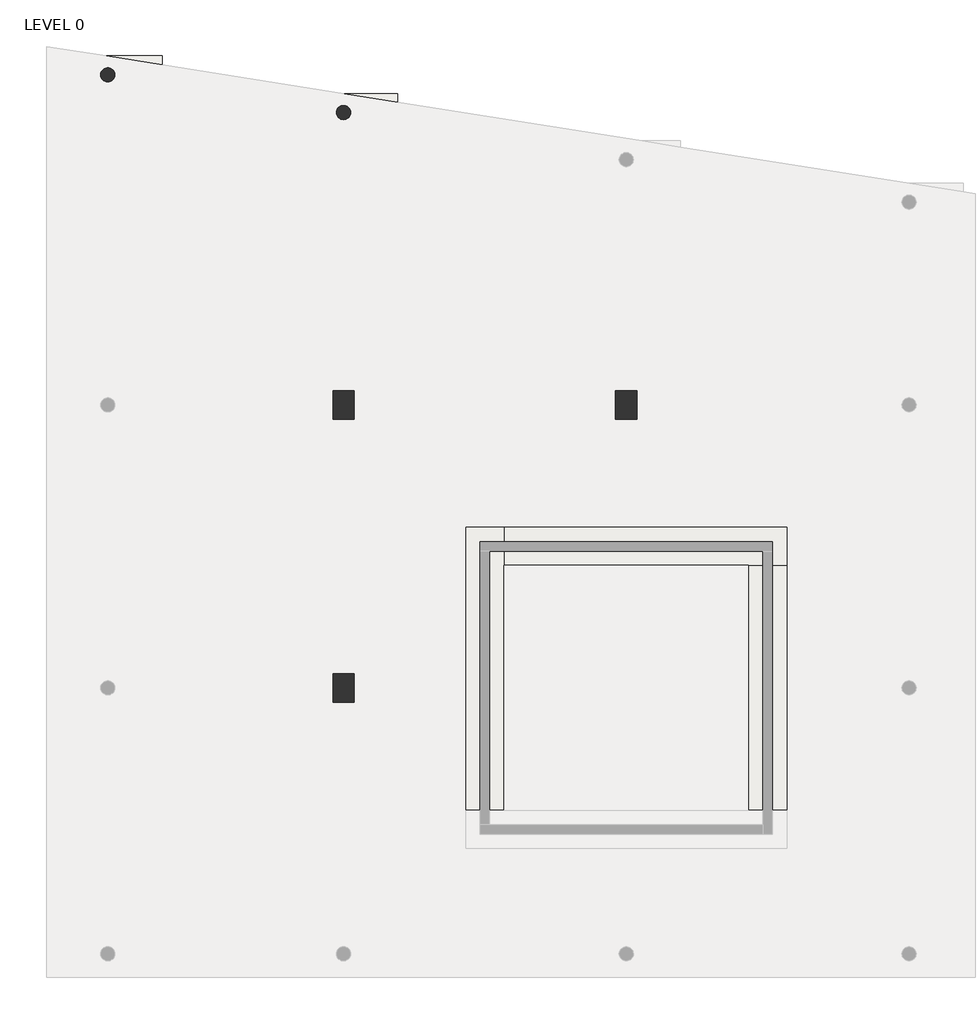
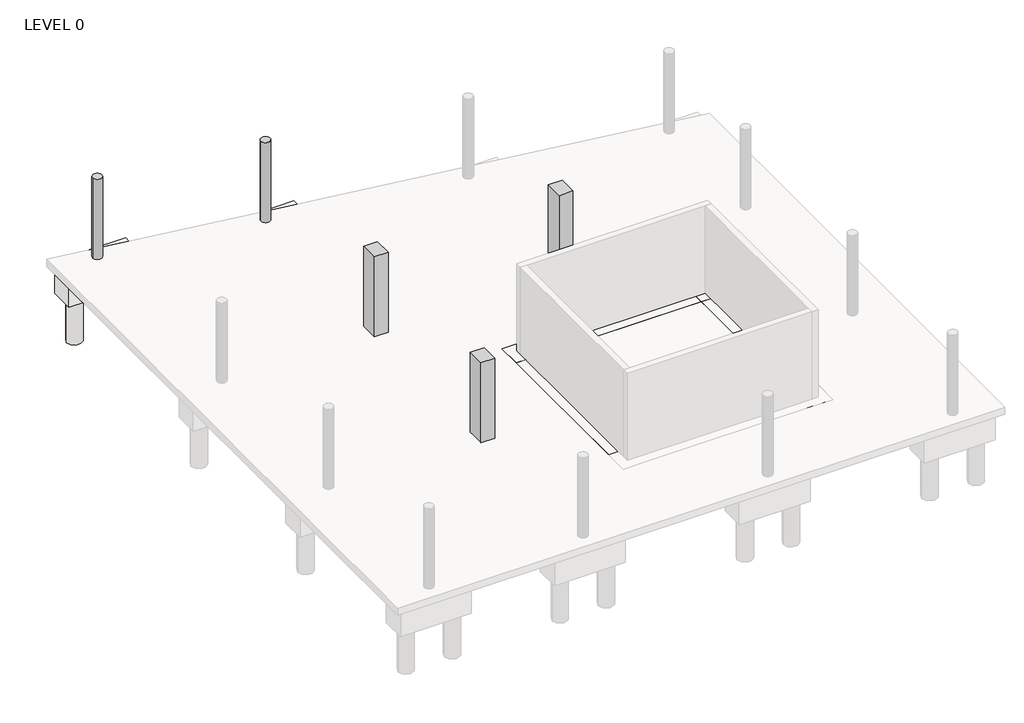
# One storey, part 2 of 3: 15 slabs, 5 columns, 3 footings.
"""IFC4 building model written with IfcOpenShell, lengths in millimetres."""

from ifc_helpers import new_model, si_unit, point, frame, frame_2d, origin, origin_with_axes, place, context, project, spatial, polyline, circle_curve, trimmed, segment, composite_curve, outline, extrude, faceted_brep, element, save
from ifc_brep_helpers import plane_surface, cylinder_surface, revolved_surface, advanced_brep

model = new_model("IFC4")

# Units and contexts
model_context = context("Model", 3, world=origin())
ifc_project = project(units=[si_unit("LENGTHUNIT", "METRE", prefix="MILLI")], contexts=[model_context])

# Site, building, storey
site = spatial("IfcSite", under=ifc_project)
building = spatial("IfcBuilding", under=site)
storey = spatial("IfcBuildingStorey", under=building, Name="LEVEL 0", Elevation=0.0)

# Columns
placement = place(None, origin())
element("IfcColumn", 1, ObjectType="BHm_StructuralColumns_ConcreteRound : 300 Ø RC COL", at=placement, inside=storey, context=model_context, shape_type="SweptSolid", body=[
    extrude(outline(composite_curve([segment(trimmed(circle_curve(frame_2d((-11075.1680269, 20840.7845261)), 150.0), [point((-11225.1680269, 20840.7845261))], [point((-10925.1680269, 20840.7845261))], False, "CARTESIAN"), True, "CONTINUOUS"), segment(trimmed(circle_curve(frame_2d((-11075.1680269, 20840.7845261)), 150.0), [point((-10925.1680269, 20840.7845261))], [point((-11225.1680269, 20840.7845261))], False, "CARTESIAN"), True, "CONTINUOUS")], self_intersect=False)), origin_with_axes(), (0.0, 0.0, 1.0), 2750.0),
])
element("IfcColumn", 2, ObjectType="BHm_StructuralColumns_ConcreteRound : 300 Ø RC COL", at=placement, inside=storey, context=model_context, shape_type="SweptSolid", body=[
    extrude(outline(composite_curve([segment(trimmed(circle_curve(frame_2d((-16075.1680269, 21640.7845261)), 150.0), [point((-16225.1680269, 21640.7845261))], [point((-15925.1680269, 21640.7845261))], False, "CARTESIAN"), True, "CONTINUOUS"), segment(trimmed(circle_curve(frame_2d((-16075.1680269, 21640.7845261)), 150.0), [point((-15925.1680269, 21640.7845261))], [point((-16225.1680269, 21640.7845261))], False, "CARTESIAN"), True, "CONTINUOUS")], self_intersect=False)), origin_with_axes(), (0.0, 0.0, 1.0), 2750.0),
])
element("IfcColumn", 3, ObjectType="BHm_StructuralColumns_ConcreteRectangular : 450x600 RC COL", at=placement, inside=storey, context=model_context, shape_type="SweptSolid", body=[
    extrude(outline(polyline([(-10850.1680269, 14940.7845261), (-10850.1680269, 14340.7845261), (-11300.1680269, 14340.7845261), (-11300.1680269, 14940.7845261), (-10850.1680269, 14940.7845261)])), origin_with_axes(), (0.0, 0.0, 1.0), 2750.0),
])
element("IfcColumn", 4, ObjectType="BHm_StructuralColumns_ConcreteRectangular : 450x600 RC COL", at=placement, inside=storey, context=model_context, shape_type="SweptSolid", body=[
    extrude(outline(polyline([(-10850.1680269, 8940.7845261), (-10850.1680269, 8340.7845261), (-11300.1680269, 8340.7845261), (-11300.1680269, 8940.7845261), (-10850.1680269, 8940.7845261)])), origin_with_axes(), (0.0, 0.0, 1.0), 2750.0),
])
element("IfcColumn", 5, ObjectType="BHm_StructuralColumns_ConcreteRectangular : 450x600 RC COL", at=placement, inside=storey, context=model_context, shape_type="SweptSolid", body=[
    extrude(outline(polyline([(-4850.1680269, 14940.7845261), (-4850.1680269, 14340.7845261), (-5300.1680269, 14340.7845261), (-5300.1680269, 14940.7845261), (-4850.1680269, 14940.7845261)])), origin_with_axes(), (0.0, 0.0, 1.0), 2750.0),
])

# Footings
element("IfcFooting", 6, ObjectType="Wall Foundation", at=placement, inside=storey, context=model_context, shape_type="Brep", body=[
    faceted_brep([(-7670.3680269, 5235.9845261, 0.0), (-7670.3680269, 6045.5845261, 0.0), (-7670.3680269, 11235.9845261, 0.0), (-7670.3680269, 12045.5845261, 0.0), (-8479.9680269, 12045.5845261, 0.0), (-8479.9680269, 5235.9845261, 0.0), (-8479.9680269, 5235.9845261, -500.0), (-8479.9680269, 5235.9845261, -250.0), (-8479.9680269, 12045.5845261, -250.0), (-8479.9680269, 12045.5845261, -500.0), (-7670.3680269, 5235.9845261, -500.0), (-7670.3680269, 12045.5845261, -500.0)], [[[0, 1, 2, 3, 4, 5]], [[6, 7, 5, 4, 8, 9]], [[10, 6, 9, 11]], [[0, 10, 11, 3, 2, 1]], [[4, 3, 11, 9, 8]], [[0, 5, 7, 6, 10]]]),
])
element("IfcFooting", 7, ObjectType="Wall Foundation", at=placement, inside=storey, context=model_context, shape_type="Brep", body=[
    faceted_brep([(-8479.9680269, 11235.9845261, 0.0), (-7670.3680269, 11235.9845261, 0.0), (-2479.9680269, 11235.9845261, 0.0), (-1670.3680269, 11235.9845261, 0.0), (-1670.3680269, 12045.5845261, 0.0), (-8479.9680269, 12045.5845261, 0.0), (-8479.9680269, 12045.5845261, -500.0), (-8479.9680269, 12045.5845261, -250.0), (-1670.3680269, 12045.5845261, -250.0), (-1670.3680269, 12045.5845261, -500.0), (-8479.9680269, 11235.9845261, -500.0), (-1670.3680269, 11235.9845261, -500.0)], [[[0, 1, 2, 3, 4, 5]], [[6, 7, 5, 4, 8, 9]], [[10, 6, 9, 11]], [[0, 10, 11, 3, 2, 1]], [[0, 5, 7, 6, 10]], [[4, 3, 11, 9, 8]]]),
])
element("IfcFooting", 8, ObjectType="Wall Foundation", at=placement, inside=storey, context=model_context, shape_type="Brep", body=[
    faceted_brep([(-2479.9680269, 12045.5845261, 0.0), (-2479.9680269, 11235.9845261, 0.0), (-2479.9680269, 6045.5845261, 0.0), (-2479.9680269, 5235.9845261, 0.0), (-1670.3680269, 5235.9845261, 0.0), (-1670.3680269, 12045.5845261, 0.0), (-1670.3680269, 12045.5845261, -500.0), (-1670.3680269, 12045.5845261, -250.0), (-1670.3680269, 5235.9845261, -250.0), (-1670.3680269, 5235.9845261, -500.0), (-2479.9680269, 12045.5845261, -500.0), (-2479.9680269, 5235.9845261, -500.0)], [[[0, 1, 2, 3, 4, 5]], [[6, 7, 5, 4, 8, 9]], [[10, 6, 9, 11]], [[0, 10, 11, 3, 2, 1]], [[0, 5, 7, 6, 10]], [[4, 3, 11, 9, 8]]]),
])

# Slabs
element("IfcSlab", 9, ObjectType="BHm_StructuralFoundations_RC-2PileCap : 500Ø R.C. 2-PILE CAP", at=placement, inside=storey, context=model_context, shape_type="AdvancedBrep", body=[
    advanced_brep(
    [(-9925.1680269, 15040.7845261, -1100.0), (-9925.1680269, 14240.7845261, -1100.0), (-12225.1680269, 14240.7845261, -1100.0), (-12225.1680269, 15040.7845261, -1100.0), (-12075.1680269, 14640.7845261, -1100.0), (-11575.1680269, 14640.7845261, -1100.0), (-10575.1680269, 14640.7845261, -1100.0), (-10075.1680269, 14640.7845261, -1100.0), (-12225.1680269, 15040.7845261, -250.0), (-9925.1680269, 15040.7845261, -250.0), (-12225.1680269, 14240.7845261, -250.0), (-9925.1680269, 14240.7845261, -250.0), (-10575.1680269, 14640.7845261, -1025.0), (-10075.1680269, 14640.7845261, -1025.0), (-12075.1680269, 14640.7845261, -1025.0), (-11575.1680269, 14640.7845261, -1025.0)],
    [
        (0, 1),
        (1, 2),
        (2, 3),
        (3, 0),
        (4, 5, circle_curve(frame((-11825.1680269, 14640.7845261, -1100.0), z_axis=(0.0, 0.0, 1.0), x_axis=(1.0, 0.0, 0.0)), 250.0)),
        (5, 4, circle_curve(frame((-11825.1680269, 14640.7845261, -1100.0), z_axis=(0.0, 0.0, 1.0), x_axis=(1.0, 0.0, 0.0)), 250.0)),
        (6, 7, circle_curve(frame((-10325.1680269, 14640.7845261, -1100.0), z_axis=(0.0, 0.0, 1.0), x_axis=(1.0, 0.0, 0.0)), 250.0)),
        (7, 6, circle_curve(frame((-10325.1680269, 14640.7845261, -1100.0), z_axis=(0.0, 0.0, 1.0), x_axis=(1.0, 0.0, 0.0)), 250.0)),
        (3, 8),
        (8, 9),
        (9, 0),
        (2, 10),
        (10, 8),
        (1, 11),
        (11, 10),
        (9, 11),
        (12, 13, circle_curve(frame((-10325.1680269, 14640.7845261, -1025.0), z_axis=(0.0, 0.0, -1.0), x_axis=(1.0, 0.0, 0.0)), 250.0)),
        (13, 12, circle_curve(frame((-10325.1680269, 14640.7845261, -1025.0), z_axis=(0.0, 0.0, -1.0), x_axis=(1.0, 0.0, 0.0)), 250.0)),
        (4, 14),
        (14, 15, circle_curve(frame((-11825.1680269, 14640.7845261, -1025.0), z_axis=(0.0, 0.0, 1.0), x_axis=(1.0, 0.0, 0.0)), 250.0)),
        (15, 5),
        (15, 14, circle_curve(frame((-11825.1680269, 14640.7845261, -1025.0), z_axis=(0.0, 0.0, 1.0), x_axis=(1.0, 0.0, 0.0)), 250.0)),
        (6, 12),
        (13, 7),
    ],
    [
        plane_surface(frame((-12225.1680269, 15040.7845261, -1100.0), z_axis=(0.0, 0.0, -1.0), x_axis=(1.0, 0.0, 0.0))),
        plane_surface(frame((-9925.1680269, 15040.7845261, 0.0), z_axis=(0.0, 1.0, 0.0), x_axis=(0.0, 0.0, -1.0))),
        plane_surface(frame((-12225.1680269, 15040.7845261, 0.0), z_axis=(-1.0, 0.0, 0.0), x_axis=(0.0, 0.0, -1.0))),
        plane_surface(frame((-12225.1680269, 14240.7845261, 0.0), z_axis=(0.0, -1.0, 0.0), x_axis=(0.0, 0.0, -1.0))),
        plane_surface(frame((-9925.1680269, 14240.7845261, 0.0), z_axis=(1.0, 0.0, 0.0), x_axis=(0.0, 0.0, -1.0))),
        plane_surface(frame((-11575.1680269, 14640.7845261, -1025.0), z_axis=(0.0, 0.0, -1.0), x_axis=(0.0, 1.0, 0.0))),
        revolved_surface(polyline([(-11575.1680269, 14640.7845261, -1025.0), (-11575.1680269, 14640.7845261, -1100.0)]), (-11825.1680269, 14640.7845261, -1100.0), (0.0, 0.0, 1.0)),
        revolved_surface(polyline([(-10075.1680269, 14640.7845261, -1025.0), (-10075.1680269, 14640.7845261, -1100.0)]), (-10325.1680269, 14640.7845261, 0.0), (0.0, 0.0, 1.0)),
        plane_surface(frame((2324.8319731, 15140.7845261, -250.0), z_axis=(0.0, 0.0, 1.0), x_axis=(0.0, -1.0, 0.0))),
    ],
    [
        (0, [[1, 2, 3, 4], [5, 6], [7, 8]]),
        (1, [[-4, 9, 10, 11]]),
        (2, [[-3, 12, 13, -9]]),
        (3, [[-2, 14, 15, -12]]),
        (4, [[-1, -11, 16, -14]]),
        (5, [[17, 18]]),
        (6, [[-5, 19, 20, 21]]),
        (6, [[-6, -21, 22, -19]]),
        (7, [[-7, 23, -18, 24]]),
        (7, [[-8, -24, -17, -23]]),
        (8, [[-10, -13, -15, -16]]),
        (5, [[-22, -20]]),
    ],
),
])
element("IfcSlab", 10, ObjectType="BHm_StructuralFoundations_RC-Pile : 500Ø R.C. PILE", at=placement, inside=storey, context=model_context, shape_type="AdvancedBrep", body=[
    advanced_brep(
    [(-12075.1680269, 14640.7845261, -1025.0), (-11575.1680269, 14640.7845261, -1025.0), (-12075.1680269, 14640.7845261, -2600.0), (-11575.1680269, 14640.7845261, -2600.0), (-12075.1680269, 14640.7845261, -1100.0), (-11575.1680269, 14640.7845261, -1100.0)],
    [
        (0, 1, circle_curve(frame((-11825.1680269, 14640.7845261, -1025.0), z_axis=(0.0, 0.0, 1.0), x_axis=(1.0, 0.0, 0.0)), 250.0)),
        (1, 0, circle_curve(frame((-11825.1680269, 14640.7845261, -1025.0), z_axis=(0.0, 0.0, 1.0), x_axis=(1.0, 0.0, 0.0)), 250.0)),
        (2, 3, circle_curve(frame((-11825.1680269, 14640.7845261, -2600.0), z_axis=(0.0, 0.0, -1.0), x_axis=(1.0, 0.0, 0.0)), 250.0)),
        (3, 2, circle_curve(frame((-11825.1680269, 14640.7845261, -2600.0), z_axis=(0.0, 0.0, -1.0), x_axis=(1.0, 0.0, 0.0)), 250.0)),
        (0, 4),
        (4, 2),
        (3, 5),
        (5, 1),
    ],
    [
        plane_surface(frame((-11575.1680269, 14640.7845261, -1025.0), z_axis=(0.0, 0.0, 1.0), x_axis=(0.0, 1.0, 0.0))),
        plane_surface(frame((-11575.1680269, 14640.7845261, -2600.0), z_axis=(0.0, 0.0, -1.0), x_axis=(0.0, -1.0, 0.0))),
        cylinder_surface(frame((-11825.1680269, 14640.7845261, -2600.0), z_axis=(0.0, 0.0, 1.0), x_axis=(1.0, 0.0, 0.0)), 250.0),
    ],
    [
        (0, [[1, 2]]),
        (1, [[3, 4]]),
        (2, [[-1, 5, 6, -4, 7, 8]]),
        (2, [[-2, -8, -7, -3, -6, -5]]),
    ],
),
])
element("IfcSlab", 11, ObjectType="BHm_StructuralFoundations_RC-Pile : 500Ø R.C. PILE", at=placement, inside=storey, context=model_context, shape_type="AdvancedBrep", body=[
    advanced_brep(
    [(-10575.1680269, 14640.7845261, -1025.0), (-10075.1680269, 14640.7845261, -1025.0), (-10575.1680269, 14640.7845261, -2600.0), (-10075.1680269, 14640.7845261, -2600.0), (-10575.1680269, 14640.7845261, -1100.0), (-10075.1680269, 14640.7845261, -1100.0)],
    [
        (0, 1, circle_curve(frame((-10325.1680269, 14640.7845261, -1025.0), z_axis=(0.0, 0.0, 1.0), x_axis=(1.0, 0.0, 0.0)), 250.0)),
        (1, 0, circle_curve(frame((-10325.1680269, 14640.7845261, -1025.0), z_axis=(0.0, 0.0, 1.0), x_axis=(1.0, 0.0, 0.0)), 250.0)),
        (2, 3, circle_curve(frame((-10325.1680269, 14640.7845261, -2600.0), z_axis=(0.0, 0.0, -1.0), x_axis=(1.0, 0.0, 0.0)), 250.0)),
        (3, 2, circle_curve(frame((-10325.1680269, 14640.7845261, -2600.0), z_axis=(0.0, 0.0, -1.0), x_axis=(1.0, 0.0, 0.0)), 250.0)),
        (0, 4),
        (4, 2),
        (3, 5),
        (5, 1),
    ],
    [
        plane_surface(frame((-10075.1680269, 14640.7845261, -1025.0), z_axis=(0.0, 0.0, 1.0), x_axis=(0.0, 1.0, 0.0))),
        plane_surface(frame((-10075.1680269, 14640.7845261, -2600.0), z_axis=(0.0, 0.0, -1.0), x_axis=(0.0, -1.0, 0.0))),
        cylinder_surface(frame((-10325.1680269, 14640.7845261, -2600.0), z_axis=(0.0, 0.0, 1.0), x_axis=(1.0, 0.0, 0.0)), 250.0),
    ],
    [
        (0, [[1, 2]]),
        (1, [[3, 4]]),
        (2, [[-1, 5, 6, -4, 7, 8]]),
        (2, [[-2, -8, -7, -3, -6, -5]]),
    ],
),
])
element("IfcSlab", 12, ObjectType="BHm_StructuralFoundations_RC-2PileCap : 500Ø R.C. 2-PILE CAP", at=placement, inside=storey, context=model_context, shape_type="AdvancedBrep", body=[
    advanced_brep(
    [(-3925.1680269, 15040.7845261, -1100.0), (-3925.1680269, 14240.7845261, -1100.0), (-6225.1680269, 14240.7845261, -1100.0), (-6225.1680269, 15040.7845261, -1100.0), (-6075.1680269, 14640.7845261, -1100.0), (-5575.1680269, 14640.7845261, -1100.0), (-4575.1680269, 14640.7845261, -1100.0), (-4075.1680269, 14640.7845261, -1100.0), (-6225.1680269, 15040.7845261, -250.0), (-3925.1680269, 15040.7845261, -250.0), (-6225.1680269, 14240.7845261, -250.0), (-3925.1680269, 14240.7845261, -250.0), (-4575.1680269, 14640.7845261, -1025.0), (-4075.1680269, 14640.7845261, -1025.0), (-6075.1680269, 14640.7845261, -1025.0), (-5575.1680269, 14640.7845261, -1025.0)],
    [
        (0, 1),
        (1, 2),
        (2, 3),
        (3, 0),
        (4, 5, circle_curve(frame((-5825.1680269, 14640.7845261, -1100.0), z_axis=(0.0, 0.0, 1.0), x_axis=(1.0, 0.0, 0.0)), 250.0)),
        (5, 4, circle_curve(frame((-5825.1680269, 14640.7845261, -1100.0), z_axis=(0.0, 0.0, 1.0), x_axis=(1.0, 0.0, 0.0)), 250.0)),
        (6, 7, circle_curve(frame((-4325.1680269, 14640.7845261, -1100.0), z_axis=(0.0, 0.0, 1.0), x_axis=(1.0, 0.0, 0.0)), 250.0)),
        (7, 6, circle_curve(frame((-4325.1680269, 14640.7845261, -1100.0), z_axis=(0.0, 0.0, 1.0), x_axis=(1.0, 0.0, 0.0)), 250.0)),
        (3, 8),
        (8, 9),
        (9, 0),
        (2, 10),
        (10, 8),
        (1, 11),
        (11, 10),
        (9, 11),
        (12, 13, circle_curve(frame((-4325.1680269, 14640.7845261, -1025.0), z_axis=(0.0, 0.0, -1.0), x_axis=(1.0, 0.0, 0.0)), 250.0)),
        (13, 12, circle_curve(frame((-4325.1680269, 14640.7845261, -1025.0), z_axis=(0.0, 0.0, -1.0), x_axis=(1.0, 0.0, 0.0)), 250.0)),
        (4, 14),
        (14, 15, circle_curve(frame((-5825.1680269, 14640.7845261, -1025.0), z_axis=(0.0, 0.0, 1.0), x_axis=(1.0, 0.0, 0.0)), 250.0)),
        (15, 5),
        (15, 14, circle_curve(frame((-5825.1680269, 14640.7845261, -1025.0), z_axis=(0.0, 0.0, 1.0), x_axis=(1.0, 0.0, 0.0)), 250.0)),
        (6, 12),
        (13, 7),
    ],
    [
        plane_surface(frame((-6225.1680269, 15040.7845261, -1100.0), z_axis=(0.0, 0.0, -1.0), x_axis=(1.0, 0.0, 0.0))),
        plane_surface(frame((-3925.1680269, 15040.7845261, 0.0), z_axis=(0.0, 1.0, 0.0), x_axis=(0.0, 0.0, -1.0))),
        plane_surface(frame((-6225.1680269, 15040.7845261, 0.0), z_axis=(-1.0, 0.0, 0.0), x_axis=(0.0, 0.0, -1.0))),
        plane_surface(frame((-6225.1680269, 14240.7845261, 0.0), z_axis=(0.0, -1.0, 0.0), x_axis=(0.0, 0.0, -1.0))),
        plane_surface(frame((-3925.1680269, 14240.7845261, 0.0), z_axis=(1.0, 0.0, 0.0), x_axis=(0.0, 0.0, -1.0))),
        plane_surface(frame((-5575.1680269, 14640.7845261, -1025.0), z_axis=(0.0, 0.0, -1.0), x_axis=(0.0, 1.0, 0.0))),
        revolved_surface(polyline([(-5575.1680269, 14640.7845261, -1025.0), (-5575.1680269, 14640.7845261, -1100.0)]), (-5825.1680269, 14640.7845261, -1100.0), (0.0, 0.0, 1.0)),
        revolved_surface(polyline([(-4075.1680269, 14640.7845261, -1025.0), (-4075.1680269, 14640.7845261, -1100.0)]), (-4325.1680269, 14640.7845261, 0.0), (0.0, 0.0, 1.0)),
        plane_surface(frame((2324.8319731, 15140.7845261, -250.0), z_axis=(0.0, 0.0, 1.0), x_axis=(0.0, -1.0, 0.0))),
    ],
    [
        (0, [[1, 2, 3, 4], [5, 6], [7, 8]]),
        (1, [[-4, 9, 10, 11]]),
        (2, [[-3, 12, 13, -9]]),
        (3, [[-2, 14, 15, -12]]),
        (4, [[-1, -11, 16, -14]]),
        (5, [[17, 18]]),
        (6, [[-5, 19, 20, 21]]),
        (6, [[-6, -21, 22, -19]]),
        (7, [[-7, 23, -18, 24]]),
        (7, [[-8, -24, -17, -23]]),
        (8, [[-10, -13, -15, -16]]),
        (5, [[-22, -20]]),
    ],
),
])
element("IfcSlab", 13, ObjectType="BHm_StructuralFoundations_RC-Pile : 500Ø R.C. PILE", at=placement, inside=storey, context=model_context, shape_type="AdvancedBrep", body=[
    advanced_brep(
    [(-6075.1680269, 14640.7845261, -1025.0), (-5575.1680269, 14640.7845261, -1025.0), (-6075.1680269, 14640.7845261, -2600.0), (-5575.1680269, 14640.7845261, -2600.0), (-6075.1680269, 14640.7845261, -1100.0), (-5575.1680269, 14640.7845261, -1100.0)],
    [
        (0, 1, circle_curve(frame((-5825.1680269, 14640.7845261, -1025.0), z_axis=(0.0, 0.0, 1.0), x_axis=(1.0, 0.0, 0.0)), 250.0)),
        (1, 0, circle_curve(frame((-5825.1680269, 14640.7845261, -1025.0), z_axis=(0.0, 0.0, 1.0), x_axis=(1.0, 0.0, 0.0)), 250.0)),
        (2, 3, circle_curve(frame((-5825.1680269, 14640.7845261, -2600.0), z_axis=(0.0, 0.0, -1.0), x_axis=(1.0, 0.0, 0.0)), 250.0)),
        (3, 2, circle_curve(frame((-5825.1680269, 14640.7845261, -2600.0), z_axis=(0.0, 0.0, -1.0), x_axis=(1.0, 0.0, 0.0)), 250.0)),
        (0, 4),
        (4, 2),
        (3, 5),
        (5, 1),
    ],
    [
        plane_surface(frame((-5575.1680269, 14640.7845261, -1025.0), z_axis=(0.0, 0.0, 1.0), x_axis=(0.0, 1.0, 0.0))),
        plane_surface(frame((-5575.1680269, 14640.7845261, -2600.0), z_axis=(0.0, 0.0, -1.0), x_axis=(0.0, -1.0, 0.0))),
        cylinder_surface(frame((-5825.1680269, 14640.7845261, -2600.0), z_axis=(0.0, 0.0, 1.0), x_axis=(1.0, 0.0, 0.0)), 250.0),
    ],
    [
        (0, [[1, 2]]),
        (1, [[3, 4]]),
        (2, [[-1, 5, 6, -4, 7, 8]]),
        (2, [[-2, -8, -7, -3, -6, -5]]),
    ],
),
])
element("IfcSlab", 14, ObjectType="BHm_StructuralFoundations_RC-Pile : 500Ø R.C. PILE", at=placement, inside=storey, context=model_context, shape_type="AdvancedBrep", body=[
    advanced_brep(
    [(-4575.1680269, 14640.7845261, -1025.0), (-4075.1680269, 14640.7845261, -1025.0), (-4575.1680269, 14640.7845261, -2600.0), (-4075.1680269, 14640.7845261, -2600.0), (-4575.1680269, 14640.7845261, -1100.0), (-4075.1680269, 14640.7845261, -1100.0)],
    [
        (0, 1, circle_curve(frame((-4325.1680269, 14640.7845261, -1025.0), z_axis=(0.0, 0.0, 1.0), x_axis=(1.0, 0.0, 0.0)), 250.0)),
        (1, 0, circle_curve(frame((-4325.1680269, 14640.7845261, -1025.0), z_axis=(0.0, 0.0, 1.0), x_axis=(1.0, 0.0, 0.0)), 250.0)),
        (2, 3, circle_curve(frame((-4325.1680269, 14640.7845261, -2600.0), z_axis=(0.0, 0.0, -1.0), x_axis=(1.0, 0.0, 0.0)), 250.0)),
        (3, 2, circle_curve(frame((-4325.1680269, 14640.7845261, -2600.0), z_axis=(0.0, 0.0, -1.0), x_axis=(1.0, 0.0, 0.0)), 250.0)),
        (0, 4),
        (4, 2),
        (3, 5),
        (5, 1),
    ],
    [
        plane_surface(frame((-4075.1680269, 14640.7845261, -1025.0), z_axis=(0.0, 0.0, 1.0), x_axis=(0.0, 1.0, 0.0))),
        plane_surface(frame((-4075.1680269, 14640.7845261, -2600.0), z_axis=(0.0, 0.0, -1.0), x_axis=(0.0, -1.0, 0.0))),
        cylinder_surface(frame((-4325.1680269, 14640.7845261, -2600.0), z_axis=(0.0, 0.0, 1.0), x_axis=(1.0, 0.0, 0.0)), 250.0),
    ],
    [
        (0, [[1, 2]]),
        (1, [[3, 4]]),
        (2, [[-1, 5, 6, -4, 7, 8]]),
        (2, [[-2, -8, -7, -3, -6, -5]]),
    ],
),
])
element("IfcSlab", 15, ObjectType="BHm_StructuralFoundations_RC-2PileCap : 500Ø R.C. 2-PILE CAP", at=placement, inside=storey, context=model_context, shape_type="AdvancedBrep", body=[
    advanced_brep(
    [(-9925.1680269, 9040.7845261, -1100.0), (-9925.1680269, 8240.7845261, -1100.0), (-12225.1680269, 8240.7845261, -1100.0), (-12225.1680269, 9040.7845261, -1100.0), (-12075.1680269, 8640.7845261, -1100.0), (-11575.1680269, 8640.7845261, -1100.0), (-10575.1680269, 8640.7845261, -1100.0), (-10075.1680269, 8640.7845261, -1100.0), (-12225.1680269, 9040.7845261, -250.0), (-9925.1680269, 9040.7845261, -250.0), (-12225.1680269, 8240.7845261, -250.0), (-9925.1680269, 8240.7845261, -250.0), (-10575.1680269, 8640.7845261, -1025.0), (-10075.1680269, 8640.7845261, -1025.0), (-12075.1680269, 8640.7845261, -1025.0), (-11575.1680269, 8640.7845261, -1025.0)],
    [
        (0, 1),
        (1, 2),
        (2, 3),
        (3, 0),
        (4, 5, circle_curve(frame((-11825.1680269, 8640.7845261, -1100.0), z_axis=(0.0, 0.0, 1.0), x_axis=(1.0, 0.0, 0.0)), 250.0)),
        (5, 4, circle_curve(frame((-11825.1680269, 8640.7845261, -1100.0), z_axis=(0.0, 0.0, 1.0), x_axis=(1.0, 0.0, 0.0)), 250.0)),
        (6, 7, circle_curve(frame((-10325.1680269, 8640.7845261, -1100.0), z_axis=(0.0, 0.0, 1.0), x_axis=(1.0, 0.0, 0.0)), 250.0)),
        (7, 6, circle_curve(frame((-10325.1680269, 8640.7845261, -1100.0), z_axis=(0.0, 0.0, 1.0), x_axis=(1.0, 0.0, 0.0)), 250.0)),
        (3, 8),
        (8, 9),
        (9, 0),
        (2, 10),
        (10, 8),
        (1, 11),
        (11, 10),
        (9, 11),
        (12, 13, circle_curve(frame((-10325.1680269, 8640.7845261, -1025.0), z_axis=(0.0, 0.0, -1.0), x_axis=(1.0, 0.0, 0.0)), 250.0)),
        (13, 12, circle_curve(frame((-10325.1680269, 8640.7845261, -1025.0), z_axis=(0.0, 0.0, -1.0), x_axis=(1.0, 0.0, 0.0)), 250.0)),
        (4, 14),
        (14, 15, circle_curve(frame((-11825.1680269, 8640.7845261, -1025.0), z_axis=(0.0, 0.0, 1.0), x_axis=(1.0, 0.0, 0.0)), 250.0)),
        (15, 5),
        (15, 14, circle_curve(frame((-11825.1680269, 8640.7845261, -1025.0), z_axis=(0.0, 0.0, 1.0), x_axis=(1.0, 0.0, 0.0)), 250.0)),
        (6, 12),
        (13, 7),
    ],
    [
        plane_surface(frame((-12225.1680269, 9040.7845261, -1100.0), z_axis=(0.0, 0.0, -1.0), x_axis=(1.0, 0.0, 0.0))),
        plane_surface(frame((-9925.1680269, 9040.7845261, 0.0), z_axis=(0.0, 1.0, 0.0), x_axis=(0.0, 0.0, -1.0))),
        plane_surface(frame((-12225.1680269, 9040.7845261, 0.0), z_axis=(-1.0, 0.0, 0.0), x_axis=(0.0, 0.0, -1.0))),
        plane_surface(frame((-12225.1680269, 8240.7845261, 0.0), z_axis=(0.0, -1.0, 0.0), x_axis=(0.0, 0.0, -1.0))),
        plane_surface(frame((-9925.1680269, 8240.7845261, 0.0), z_axis=(1.0, 0.0, 0.0), x_axis=(0.0, 0.0, -1.0))),
        plane_surface(frame((-11575.1680269, 8640.7845261, -1025.0), z_axis=(0.0, 0.0, -1.0), x_axis=(0.0, 1.0, 0.0))),
        revolved_surface(polyline([(-11575.1680269, 8640.7845261, -1025.0), (-11575.1680269, 8640.7845261, -1100.0)]), (-11825.1680269, 8640.7845261, -1100.0), (0.0, 0.0, 1.0)),
        revolved_surface(polyline([(-10075.1680269, 8640.7845261, -1025.0), (-10075.1680269, 8640.7845261, -1100.0)]), (-10325.1680269, 8640.7845261, 0.0), (0.0, 0.0, 1.0)),
        plane_surface(frame((2324.8319731, 15140.7845261, -250.0), z_axis=(0.0, 0.0, 1.0), x_axis=(0.0, -1.0, 0.0))),
    ],
    [
        (0, [[1, 2, 3, 4], [5, 6], [7, 8]]),
        (1, [[-4, 9, 10, 11]]),
        (2, [[-3, 12, 13, -9]]),
        (3, [[-2, 14, 15, -12]]),
        (4, [[-1, -11, 16, -14]]),
        (5, [[17, 18]]),
        (6, [[-5, 19, 20, 21]]),
        (6, [[-6, -21, 22, -19]]),
        (7, [[-7, 23, -18, 24]]),
        (7, [[-8, -24, -17, -23]]),
        (8, [[-10, -13, -15, -16]]),
        (5, [[-22, -20]]),
    ],
),
])
element("IfcSlab", 16, ObjectType="BHm_StructuralFoundations_RC-Pile : 500Ø R.C. PILE", at=placement, inside=storey, context=model_context, shape_type="AdvancedBrep", body=[
    advanced_brep(
    [(-12075.1680269, 8640.7845261, -1025.0), (-11575.1680269, 8640.7845261, -1025.0), (-12075.1680269, 8640.7845261, -2600.0), (-11575.1680269, 8640.7845261, -2600.0), (-12075.1680269, 8640.7845261, -1100.0), (-11575.1680269, 8640.7845261, -1100.0)],
    [
        (0, 1, circle_curve(frame((-11825.1680269, 8640.7845261, -1025.0), z_axis=(0.0, 0.0, 1.0), x_axis=(1.0, 0.0, 0.0)), 250.0)),
        (1, 0, circle_curve(frame((-11825.1680269, 8640.7845261, -1025.0), z_axis=(0.0, 0.0, 1.0), x_axis=(1.0, 0.0, 0.0)), 250.0)),
        (2, 3, circle_curve(frame((-11825.1680269, 8640.7845261, -2600.0), z_axis=(0.0, 0.0, -1.0), x_axis=(1.0, 0.0, 0.0)), 250.0)),
        (3, 2, circle_curve(frame((-11825.1680269, 8640.7845261, -2600.0), z_axis=(0.0, 0.0, -1.0), x_axis=(1.0, 0.0, 0.0)), 250.0)),
        (0, 4),
        (4, 2),
        (3, 5),
        (5, 1),
    ],
    [
        plane_surface(frame((-11575.1680269, 8640.7845261, -1025.0), z_axis=(0.0, 0.0, 1.0), x_axis=(0.0, 1.0, 0.0))),
        plane_surface(frame((-11575.1680269, 8640.7845261, -2600.0), z_axis=(0.0, 0.0, -1.0), x_axis=(0.0, -1.0, 0.0))),
        cylinder_surface(frame((-11825.1680269, 8640.7845261, -2600.0), z_axis=(0.0, 0.0, 1.0), x_axis=(1.0, 0.0, 0.0)), 250.0),
    ],
    [
        (0, [[1, 2]]),
        (1, [[3, 4]]),
        (2, [[-1, 5, 6, -4, 7, 8]]),
        (2, [[-2, -8, -7, -3, -6, -5]]),
    ],
),
])
element("IfcSlab", 17, ObjectType="BHm_StructuralFoundations_RC-Pile : 500Ø R.C. PILE", at=placement, inside=storey, context=model_context, shape_type="AdvancedBrep", body=[
    advanced_brep(
    [(-10575.1680269, 8640.7845261, -1025.0), (-10075.1680269, 8640.7845261, -1025.0), (-10575.1680269, 8640.7845261, -2600.0), (-10075.1680269, 8640.7845261, -2600.0), (-10575.1680269, 8640.7845261, -1100.0), (-10075.1680269, 8640.7845261, -1100.0)],
    [
        (0, 1, circle_curve(frame((-10325.1680269, 8640.7845261, -1025.0), z_axis=(0.0, 0.0, 1.0), x_axis=(1.0, 0.0, 0.0)), 250.0)),
        (1, 0, circle_curve(frame((-10325.1680269, 8640.7845261, -1025.0), z_axis=(0.0, 0.0, 1.0), x_axis=(1.0, 0.0, 0.0)), 250.0)),
        (2, 3, circle_curve(frame((-10325.1680269, 8640.7845261, -2600.0), z_axis=(0.0, 0.0, -1.0), x_axis=(1.0, 0.0, 0.0)), 250.0)),
        (3, 2, circle_curve(frame((-10325.1680269, 8640.7845261, -2600.0), z_axis=(0.0, 0.0, -1.0), x_axis=(1.0, 0.0, 0.0)), 250.0)),
        (0, 4),
        (4, 2),
        (3, 5),
        (5, 1),
    ],
    [
        plane_surface(frame((-10075.1680269, 8640.7845261, -1025.0), z_axis=(0.0, 0.0, 1.0), x_axis=(0.0, 1.0, 0.0))),
        plane_surface(frame((-10075.1680269, 8640.7845261, -2600.0), z_axis=(0.0, 0.0, -1.0), x_axis=(0.0, -1.0, 0.0))),
        cylinder_surface(frame((-10325.1680269, 8640.7845261, -2600.0), z_axis=(0.0, 0.0, 1.0), x_axis=(1.0, 0.0, 0.0)), 250.0),
    ],
    [
        (0, [[1, 2]]),
        (1, [[3, 4]]),
        (2, [[-1, 5, 6, -4, 7, 8]]),
        (2, [[-2, -8, -7, -3, -6, -5]]),
    ],
),
])
element("IfcSlab", 18, ObjectType="BHm_StructuralFoundations_RC-Pile : 500Ø R.C. PILE", at=placement, inside=storey, context=model_context, shape_type="AdvancedBrep", body=[
    advanced_brep(
    [(-15575.1680269, 14640.7845261, -1025.0), (-15075.1680269, 14640.7845261, -1025.0), (-15575.1680269, 14640.7845261, -2600.0), (-15075.1680269, 14640.7845261, -2600.0), (-15575.1680269, 14640.7845261, -1100.0), (-15075.1680269, 14640.7845261, -1100.0)],
    [
        (0, 1, circle_curve(frame((-15325.1680269, 14640.7845261, -1025.0), z_axis=(0.0, 0.0, 1.0), x_axis=(1.0, 0.0, 0.0)), 250.0)),
        (1, 0, circle_curve(frame((-15325.1680269, 14640.7845261, -1025.0), z_axis=(0.0, 0.0, 1.0), x_axis=(1.0, 0.0, 0.0)), 250.0)),
        (2, 3, circle_curve(frame((-15325.1680269, 14640.7845261, -2600.0), z_axis=(0.0, 0.0, -1.0), x_axis=(1.0, 0.0, 0.0)), 250.0)),
        (3, 2, circle_curve(frame((-15325.1680269, 14640.7845261, -2600.0), z_axis=(0.0, 0.0, -1.0), x_axis=(1.0, 0.0, 0.0)), 250.0)),
        (0, 4),
        (4, 2),
        (3, 5),
        (5, 1),
    ],
    [
        plane_surface(frame((-15075.1680269, 14640.7845261, -1025.0), z_axis=(0.0, 0.0, 1.0), x_axis=(0.0, 1.0, 0.0))),
        plane_surface(frame((-15075.1680269, 14640.7845261, -2600.0), z_axis=(0.0, 0.0, -1.0), x_axis=(0.0, -1.0, 0.0))),
        cylinder_surface(frame((-15325.1680269, 14640.7845261, -2600.0), z_axis=(0.0, 0.0, 1.0), x_axis=(1.0, 0.0, 0.0)), 250.0),
    ],
    [
        (0, [[1, 2]]),
        (1, [[3, 4]]),
        (2, [[-1, 5, 6, -4, 7, 8]]),
        (2, [[-2, -8, -7, -3, -6, -5]]),
    ],
),
])
element("IfcSlab", 19, ObjectType="BHm_StructuralFoundations_RC-Pile : 500Ø R.C. PILE", at=placement, inside=storey, context=model_context, shape_type="AdvancedBrep", body=[
    advanced_brep(
    [(-15575.1680269, 8640.7845261, -1025.0), (-15075.1680269, 8640.7845261, -1025.0), (-15575.1680269, 8640.7845261, -2600.0), (-15075.1680269, 8640.7845261, -2600.0), (-15575.1680269, 8640.7845261, -1100.0), (-15075.1680269, 8640.7845261, -1100.0)],
    [
        (0, 1, circle_curve(frame((-15325.1680269, 8640.7845261, -1025.0), z_axis=(0.0, 0.0, 1.0), x_axis=(1.0, 0.0, 0.0)), 250.0)),
        (1, 0, circle_curve(frame((-15325.1680269, 8640.7845261, -1025.0), z_axis=(0.0, 0.0, 1.0), x_axis=(1.0, 0.0, 0.0)), 250.0)),
        (2, 3, circle_curve(frame((-15325.1680269, 8640.7845261, -2600.0), z_axis=(0.0, 0.0, -1.0), x_axis=(1.0, 0.0, 0.0)), 250.0)),
        (3, 2, circle_curve(frame((-15325.1680269, 8640.7845261, -2600.0), z_axis=(0.0, 0.0, -1.0), x_axis=(1.0, 0.0, 0.0)), 250.0)),
        (0, 4),
        (4, 2),
        (3, 5),
        (5, 1),
    ],
    [
        plane_surface(frame((-15075.1680269, 8640.7845261, -1025.0), z_axis=(0.0, 0.0, 1.0), x_axis=(0.0, 1.0, 0.0))),
        plane_surface(frame((-15075.1680269, 8640.7845261, -2600.0), z_axis=(0.0, 0.0, -1.0), x_axis=(0.0, -1.0, 0.0))),
        cylinder_surface(frame((-15325.1680269, 8640.7845261, -2600.0), z_axis=(0.0, 0.0, 1.0), x_axis=(1.0, 0.0, 0.0)), 250.0),
    ],
    [
        (0, [[1, 2]]),
        (1, [[3, 4]]),
        (2, [[-1, 5, 6, -4, 7, 8]]),
        (2, [[-2, -8, -7, -3, -6, -5]]),
    ],
),
])
element("IfcSlab", 20, ObjectType="BHm_StructuralFoundations_RC-2PileCap : 500Ø R.C. 2-PILE CAP", at=placement, inside=storey, context=model_context, shape_type="AdvancedBrep", body=[
    advanced_brep(
    [(-9925.1680269, 21240.7845261, 0.0), (-11061.4165123, 21240.7845261, 0.0), (-9925.1680269, 21060.8204456, 0.0), (-9925.1680269, 21240.7845261, -1100.0), (-9925.1680269, 20440.7845261, -1100.0), (-12225.1680269, 20440.7845261, -1100.0), (-12225.1680269, 21240.7845261, -1100.0), (-12075.1680269, 20840.7845261, -1100.0), (-11575.1680269, 20840.7845261, -1100.0), (-10575.1680269, 20840.7845261, -1100.0), (-10075.1680269, 20840.7845261, -1100.0), (-12225.1680269, 21240.7845261, -250.0), (-11061.4165123, 21240.7845261, -250.0), (-12225.1680269, 20440.7845261, -250.0), (-9925.1680269, 20440.7845261, -250.0), (-9925.1680269, 21060.8204456, -250.0), (-10575.1680269, 20840.7845261, -1025.0), (-10075.1680269, 20840.7845261, -1025.0), (-12075.1680269, 20840.7845261, -1025.0), (-11575.1680269, 20840.7845261, -1025.0)],
    [
        (0, 1),
        (1, 2),
        (2, 0),
        (3, 4),
        (4, 5),
        (5, 6),
        (6, 3),
        (7, 8, circle_curve(frame((-11825.1680269, 20840.7845261, -1100.0), z_axis=(0.0, 0.0, 1.0), x_axis=(1.0, 0.0, 0.0)), 250.0)),
        (8, 7, circle_curve(frame((-11825.1680269, 20840.7845261, -1100.0), z_axis=(0.0, 0.0, 1.0), x_axis=(1.0, 0.0, 0.0)), 250.0)),
        (9, 10, circle_curve(frame((-10325.1680269, 20840.7845261, -1100.0), z_axis=(0.0, 0.0, 1.0), x_axis=(1.0, 0.0, 0.0)), 250.0)),
        (10, 9, circle_curve(frame((-10325.1680269, 20840.7845261, -1100.0), z_axis=(0.0, 0.0, 1.0), x_axis=(1.0, 0.0, 0.0)), 250.0)),
        (6, 11),
        (11, 12),
        (12, 1),
        (0, 3),
        (5, 13),
        (13, 11),
        (4, 14),
        (14, 13),
        (2, 15),
        (15, 14),
        (16, 17, circle_curve(frame((-10325.1680269, 20840.7845261, -1025.0), z_axis=(0.0, 0.0, -1.0), x_axis=(1.0, 0.0, 0.0)), 250.0)),
        (17, 16, circle_curve(frame((-10325.1680269, 20840.7845261, -1025.0), z_axis=(0.0, 0.0, -1.0), x_axis=(1.0, 0.0, 0.0)), 250.0)),
        (7, 18),
        (18, 19, circle_curve(frame((-11825.1680269, 20840.7845261, -1025.0), z_axis=(0.0, 0.0, 1.0), x_axis=(1.0, 0.0, 0.0)), 250.0)),
        (19, 8),
        (19, 18, circle_curve(frame((-11825.1680269, 20840.7845261, -1025.0), z_axis=(0.0, 0.0, 1.0), x_axis=(1.0, 0.0, 0.0)), 250.0)),
        (9, 16),
        (17, 10),
        (15, 12),
    ],
    [
        plane_surface(frame((-12225.1680269, 21240.7845261, 0.0), z_axis=(0.0, 0.0, 1.0), x_axis=(-1.0, 0.0, 0.0))),
        plane_surface(frame((-12225.1680269, 21240.7845261, -1100.0), z_axis=(0.0, 0.0, -1.0), x_axis=(1.0, 0.0, 0.0))),
        plane_surface(frame((-9925.1680269, 21240.7845261, 0.0), z_axis=(0.0, 1.0, 0.0), x_axis=(0.0, 0.0, -1.0))),
        plane_surface(frame((-12225.1680269, 21240.7845261, 0.0), z_axis=(-1.0, 0.0, 0.0), x_axis=(0.0, 0.0, -1.0))),
        plane_surface(frame((-12225.1680269, 20440.7845261, 0.0), z_axis=(0.0, -1.0, 0.0), x_axis=(0.0, 0.0, -1.0))),
        plane_surface(frame((-9925.1680269, 20440.7845261, 0.0), z_axis=(1.0, 0.0, 0.0), x_axis=(0.0, 0.0, -1.0))),
        plane_surface(frame((-11575.1680269, 20840.7845261, -1025.0), z_axis=(0.0, 0.0, -1.0), x_axis=(0.0, 1.0, 0.0))),
        revolved_surface(polyline([(-11575.1680269, 20840.7845261, -1025.0), (-11575.1680269, 20840.7845261, -1100.0)]), (-11825.1680269, 20840.7845261, -1100.0), (0.0, 0.0, 1.0)),
        revolved_surface(polyline([(-10075.1680269, 20840.7845261, -1025.0), (-10075.1680269, 20840.7845261, -1100.0)]), (-10325.1680269, 20840.7845261, 0.0), (0.0, 0.0, 1.0)),
        plane_surface(frame((2324.8319731, 15140.7845261, -250.0), z_axis=(0.0, 0.0, 1.0), x_axis=(0.0, -1.0, 0.0))),
        plane_surface(frame((-17375.1680269, 22240.7845261, -250.0), z_axis=(-0.15643446504023414, -0.9876883405951372, 0.0), x_axis=(0.0, 0.0, 1.0))),
    ],
    [
        (0, [[1, 2, 3]]),
        (1, [[4, 5, 6, 7], [8, 9], [10, 11]]),
        (2, [[-7, 12, 13, 14, -1, 15]]),
        (3, [[-6, 16, 17, -12]]),
        (4, [[-5, 18, 19, -16]]),
        (5, [[-4, -15, -3, 20, 21, -18]]),
        (6, [[22, 23]]),
        (7, [[-8, 24, 25, 26]]),
        (7, [[-9, -26, 27, -24]]),
        (8, [[-10, 28, -23, 29]]),
        (8, [[-11, -29, -22, -28]]),
        (9, [[30, -13, -17, -19, -21]]),
        (10, [[-30, -20, -2, -14]]),
        (6, [[-27, -25]]),
    ],
),
])
element("IfcSlab", 21, ObjectType="BHm_StructuralFoundations_RC-2PileCap : 500Ø R.C. 2-PILE CAP", at=placement, inside=storey, context=model_context, shape_type="AdvancedBrep", body=[
    advanced_brep(
    [(-14925.1680269, 22040.7845261, 0.0), (-16112.417724, 22040.7845261, 0.0), (-14925.1680269, 21852.7426473, 0.0), (-14925.1680269, 22040.7845261, -1100.0), (-14925.1680269, 21240.7845261, -1100.0), (-17225.1680269, 21240.7845261, -1100.0), (-17225.1680269, 22040.7845261, -1100.0), (-17075.1680269, 21640.7845261, -1100.0), (-16575.1680269, 21640.7845261, -1100.0), (-15575.1680269, 21640.7845261, -1100.0), (-15075.1680269, 21640.7845261, -1100.0), (-17225.1680269, 22040.7845261, -250.0), (-16112.417724, 22040.7845261, -250.0), (-17225.1680269, 21240.7845261, -250.0), (-14925.1680269, 21240.7845261, -250.0), (-14925.1680269, 21852.7426473, -250.0), (-15575.1680269, 21640.7845261, -1025.0), (-15075.1680269, 21640.7845261, -1025.0), (-17075.1680269, 21640.7845261, -1025.0), (-16575.1680269, 21640.7845261, -1025.0)],
    [
        (0, 1),
        (1, 2),
        (2, 0),
        (3, 4),
        (4, 5),
        (5, 6),
        (6, 3),
        (7, 8, circle_curve(frame((-16825.1680269, 21640.7845261, -1100.0), z_axis=(0.0, 0.0, 1.0), x_axis=(1.0, 0.0, 0.0)), 250.0)),
        (8, 7, circle_curve(frame((-16825.1680269, 21640.7845261, -1100.0), z_axis=(0.0, 0.0, 1.0), x_axis=(1.0, 0.0, 0.0)), 250.0)),
        (9, 10, circle_curve(frame((-15325.1680269, 21640.7845261, -1100.0), z_axis=(0.0, 0.0, 1.0), x_axis=(1.0, 0.0, 0.0)), 250.0)),
        (10, 9, circle_curve(frame((-15325.1680269, 21640.7845261, -1100.0), z_axis=(0.0, 0.0, 1.0), x_axis=(1.0, 0.0, 0.0)), 250.0)),
        (6, 11),
        (11, 12),
        (12, 1),
        (0, 3),
        (5, 13),
        (13, 11),
        (4, 14),
        (14, 13),
        (2, 15),
        (15, 14),
        (16, 17, circle_curve(frame((-15325.1680269, 21640.7845261, -1025.0), z_axis=(0.0, 0.0, -1.0), x_axis=(1.0, 0.0, 0.0)), 250.0)),
        (17, 16, circle_curve(frame((-15325.1680269, 21640.7845261, -1025.0), z_axis=(0.0, 0.0, -1.0), x_axis=(1.0, 0.0, 0.0)), 250.0)),
        (7, 18),
        (18, 19, circle_curve(frame((-16825.1680269, 21640.7845261, -1025.0), z_axis=(0.0, 0.0, 1.0), x_axis=(1.0, 0.0, 0.0)), 250.0)),
        (19, 8),
        (19, 18, circle_curve(frame((-16825.1680269, 21640.7845261, -1025.0), z_axis=(0.0, 0.0, 1.0), x_axis=(1.0, 0.0, 0.0)), 250.0)),
        (9, 16),
        (17, 10),
        (15, 12),
    ],
    [
        plane_surface(frame((-17225.1680269, 22040.7845261, 0.0), z_axis=(0.0, 0.0, 1.0), x_axis=(-1.0, 0.0, 0.0))),
        plane_surface(frame((-17225.1680269, 22040.7845261, -1100.0), z_axis=(0.0, 0.0, -1.0), x_axis=(1.0, 0.0, 0.0))),
        plane_surface(frame((-14925.1680269, 22040.7845261, 0.0), z_axis=(0.0, 1.0, 0.0), x_axis=(0.0, 0.0, -1.0))),
        plane_surface(frame((-17225.1680269, 22040.7845261, 0.0), z_axis=(-1.0, 0.0, 0.0), x_axis=(0.0, 0.0, -1.0))),
        plane_surface(frame((-17225.1680269, 21240.7845261, 0.0), z_axis=(0.0, -1.0, 0.0), x_axis=(0.0, 0.0, -1.0))),
        plane_surface(frame((-14925.1680269, 21240.7845261, 0.0), z_axis=(1.0, 0.0, 0.0), x_axis=(0.0, 0.0, -1.0))),
        plane_surface(frame((-16575.1680269, 21640.7845261, -1025.0), z_axis=(0.0, 0.0, -1.0), x_axis=(0.0, 1.0, 0.0))),
        revolved_surface(polyline([(-16575.1680269, 21640.7845261, -1025.0), (-16575.1680269, 21640.7845261, -1100.0)]), (-16825.1680269, 21640.7845261, -1100.0), (0.0, 0.0, 1.0)),
        revolved_surface(polyline([(-15075.1680269, 21640.7845261, -1025.0), (-15075.1680269, 21640.7845261, -1100.0)]), (-15325.1680269, 21640.7845261, 0.0), (0.0, 0.0, 1.0)),
        plane_surface(frame((2324.8319731, 15140.7845261, -250.0), z_axis=(0.0, 0.0, 1.0), x_axis=(0.0, -1.0, 0.0))),
        plane_surface(frame((-17375.1680269, 22240.7845261, -250.0), z_axis=(-0.15643446504023414, -0.9876883405951372, 0.0), x_axis=(0.0, 0.0, 1.0))),
    ],
    [
        (0, [[1, 2, 3]]),
        (1, [[4, 5, 6, 7], [8, 9], [10, 11]]),
        (2, [[-7, 12, 13, 14, -1, 15]]),
        (3, [[-6, 16, 17, -12]]),
        (4, [[-5, 18, 19, -16]]),
        (5, [[-4, -15, -3, 20, 21, -18]]),
        (6, [[22, 23]]),
        (7, [[-8, 24, 25, 26]]),
        (7, [[-9, -26, 27, -24]]),
        (8, [[-10, 28, -23, 29]]),
        (8, [[-11, -29, -22, -28]]),
        (9, [[30, -13, -17, -19, -21]]),
        (10, [[-30, -20, -2, -14]]),
        (6, [[-27, -25]]),
    ],
),
])
element("IfcSlab", 22, ObjectType="BHm_StructuralFoundations_RC-Pile : 500Ø R.C. PILE", at=placement, inside=storey, context=model_context, shape_type="AdvancedBrep", body=[
    advanced_brep(
    [(-17075.1680269, 21640.7845261, -1025.0), (-16575.1680269, 21640.7845261, -1025.0), (-17075.1680269, 21640.7845261, -2600.0), (-16575.1680269, 21640.7845261, -2600.0), (-17075.1680269, 21640.7845261, -1100.0), (-16575.1680269, 21640.7845261, -1100.0)],
    [
        (0, 1, circle_curve(frame((-16825.1680269, 21640.7845261, -1025.0), z_axis=(0.0, 0.0, 1.0), x_axis=(1.0, 0.0, 0.0)), 250.0)),
        (1, 0, circle_curve(frame((-16825.1680269, 21640.7845261, -1025.0), z_axis=(0.0, 0.0, 1.0), x_axis=(1.0, 0.0, 0.0)), 250.0)),
        (2, 3, circle_curve(frame((-16825.1680269, 21640.7845261, -2600.0), z_axis=(0.0, 0.0, -1.0), x_axis=(1.0, 0.0, 0.0)), 250.0)),
        (3, 2, circle_curve(frame((-16825.1680269, 21640.7845261, -2600.0), z_axis=(0.0, 0.0, -1.0), x_axis=(1.0, 0.0, 0.0)), 250.0)),
        (0, 4),
        (4, 2),
        (3, 5),
        (5, 1),
    ],
    [
        plane_surface(frame((-16575.1680269, 21640.7845261, -1025.0), z_axis=(0.0, 0.0, 1.0), x_axis=(0.0, 1.0, 0.0))),
        plane_surface(frame((-16575.1680269, 21640.7845261, -2600.0), z_axis=(0.0, 0.0, -1.0), x_axis=(0.0, -1.0, 0.0))),
        cylinder_surface(frame((-16825.1680269, 21640.7845261, -2600.0), z_axis=(0.0, 0.0, 1.0), x_axis=(1.0, 0.0, 0.0)), 250.0),
    ],
    [
        (0, [[1, 2]]),
        (1, [[3, 4]]),
        (2, [[-1, 5, 6, -4, 7, 8]]),
        (2, [[-2, -8, -7, -3, -6, -5]]),
    ],
),
])
element("IfcSlab", 23, ObjectType="BHm_StructuralFoundations_RC-Pile : 500Ø R.C. PILE", at=placement, inside=storey, context=model_context, shape_type="AdvancedBrep", body=[
    advanced_brep(
    [(-15575.1680269, 21640.7845261, -1025.0), (-15075.1680269, 21640.7845261, -1025.0), (-15575.1680269, 21640.7845261, -2600.0), (-15075.1680269, 21640.7845261, -2600.0), (-15575.1680269, 21640.7845261, -1100.0), (-15075.1680269, 21640.7845261, -1100.0)],
    [
        (0, 1, circle_curve(frame((-15325.1680269, 21640.7845261, -1025.0), z_axis=(0.0, 0.0, 1.0), x_axis=(1.0, 0.0, 0.0)), 250.0)),
        (1, 0, circle_curve(frame((-15325.1680269, 21640.7845261, -1025.0), z_axis=(0.0, 0.0, 1.0), x_axis=(1.0, 0.0, 0.0)), 250.0)),
        (2, 3, circle_curve(frame((-15325.1680269, 21640.7845261, -2600.0), z_axis=(0.0, 0.0, -1.0), x_axis=(1.0, 0.0, 0.0)), 250.0)),
        (3, 2, circle_curve(frame((-15325.1680269, 21640.7845261, -2600.0), z_axis=(0.0, 0.0, -1.0), x_axis=(1.0, 0.0, 0.0)), 250.0)),
        (0, 4),
        (4, 2),
        (3, 5),
        (5, 1),
    ],
    [
        plane_surface(frame((-15075.1680269, 21640.7845261, -1025.0), z_axis=(0.0, 0.0, 1.0), x_axis=(0.0, 1.0, 0.0))),
        plane_surface(frame((-15075.1680269, 21640.7845261, -2600.0), z_axis=(0.0, 0.0, -1.0), x_axis=(0.0, -1.0, 0.0))),
        cylinder_surface(frame((-15325.1680269, 21640.7845261, -2600.0), z_axis=(0.0, 0.0, 1.0), x_axis=(1.0, 0.0, 0.0)), 250.0),
    ],
    [
        (0, [[1, 2]]),
        (1, [[3, 4]]),
        (2, [[-1, 5, 6, -4, 7, 8]]),
        (2, [[-2, -8, -7, -3, -6, -5]]),
    ],
),
])

save(model, "model.ifc")

# Revit data of these elements
# Type "BHm_StructuralColumns_ConcreteRound : 300 Ø RC COL"
#   Keynote = "E"
#   b = 300.000 mm
#   BHE_Length [instance default] = 2500.000 mm
#   BHE_Diameter = 300.000 mm
#   Structural Material [instance default] = none
# Type "BHm_StructuralColumns_ConcreteRectangular : 450x600 RC COL"
#   Keynote = "E"
#   b = 450.000 mm
#   h = 600.000 mm
#   BHE_Width = 450.000 mm
#   BHE_Length [instance default] = 2500.000 mm
#   BHE_Height = 600.000 mm
#   Structural Material [instance default] = none
# Type "BHm_StructuralFoundations_RC-2PileCap : 500Ø R.C. 2-PILE CAP"
#   BHE_Tension/Compression [instance default] = ""
#   BHE_SLS Min Vertical LL (kN) [instance default] = ""
#   BHE_SLS Min Vertical DL (kN) [instance default] = ""
#   BHE_SLS Max Vertical LL (kN) [instance default] = ""
#   BHE_SLS Max Vertical DL (kN) [instance default] = ""
#   BHE_SLS Max ML (kNm) [instance default] = ""
#   BHE_SLS Geo Short Term Heave Action (kN) [instance default] = ""
#   BHE_SLS Geo Max Moment Load (kNm) [instance default] = ""
#   BHE_SLS Geo Max Horizontal Load (kN) [instance default] = ""
#   BHE_SLS Geo Max Groundwater Pressure Action (kN) [instance default] = ""
#   BHE_SLS Geo Long Term Heave Action (kN) [instance default] = ""
#   BHE_Min Vertical Steel (mm²) [instance default] = ""
#   BHE_Curtailment Level (mOD) [instance default] = ""
#   bhe_k = 3
#   Width = 800.000 mm
#   bhe_Void Position Top = -1025.000 mm
#   Pile Spacing = 1500.000 mm
#   bhe_Pile Insertion Vertical Offset = -1100.000 mm
#   Length = 2300.000 mm
#   Default Elevation = 1219.200 mm
#   BHE_Width = 800.000 mm
#   BHE_Radius = 250.000 mm
#   BHE_Pile Embedment Numerical = 75
#   BHE_Pile Embedment = 75.000 mm
#   BHE_Pile Edge Distance = 150.000 mm
#   BHE_Pile Depth Numerical [instance default] = 1500
#   BHE_Pile Depth [instance default] = 1500.000 mm
#   BHE_Length = 2300.000 mm
#   BHE_Diameter = 500.000 mm
#   BHE_Depth = 1100.000 mm
#   bhe_Pile Size = BHm_StructuralFoundations_RC-Pile : 500Ø R.C. PILE
#   Structural Material = none
#   Assembly Code = ""
# Type "BHm_StructuralFoundations_RC-Pile : 500Ø R.C. PILE"
#   Type Comments = "500Ø R.C. PILE"
#   Keynote = "500Ø R.C. PILE"
#   BHE_Tension/Compression [instance default] = ""
#   BHE_SLS Min Vertical LL (kN) [instance default] = ""
#   BHE_SLS Min Vertical DL (kN) [instance default] = ""
#   BHE_SLS Max Vertical LL (kN) [instance default] = ""
#   BHE_SLS Max Vertical DL (kN) [instance default] = ""
#   BHE_SLS Max ML (kNm) [instance default] = ""
#   BHE_SLS Geo Short Term Heave Action (kN) [instance default] = ""
#   BHE_SLS Geo Max Moment Load (kNm) [instance default] = ""
#   BHE_SLS Geo Max Horizontal Load (kN) [instance default] = ""
#   BHE_SLS Geo Max Groundwater Pressure Action (kN) [instance default] = ""
#   BHE_SLS Geo Long Term Heave Action (kN) [instance default] = ""
#   BHE_Min Vertical Steel (mm²) [instance default] = ""
#   BHE_Curtailment Level (mOD) [instance default] = ""
#   bhe_Pile Offset Line 3Ø = 1500.000 mm
#   bhe_Pile Offset Line 2.5Ø = 1250.000 mm
#   BHE_Radius = 250.000 mm
#   BHE_Pile Length [instance default] = 1575.000 mm
#   BHE_Pile Embedment Numerical [instance default] = 75
#   BHE_Pile Embedment [instance default] = 75.000 mm
#   BHE_Pile Depth Numerical [instance default] = 1500
#   BHE_Pile Depth [instance default] = 1500.000 mm
#   BHE_Diameter = 500.000 mm
#   BHE_Pile Offset Line Vis 3Ø = yes
#   BHE_Pile Offset Line Vis 2.5Ø = yes
#   BHE_Lightning Protection [instance default] = no
#   Structural Material = none
#   Description = (empty or 0)
#   Assembly Code = ""
# Elements 1, 2 (IfcColumn, "BHm_StructuralColumns_ConcreteRound : 300 Ø RC COL")
#   Comments = ""
#   Structural Material = none
#   Phase Created = New Construction
#   Materials on its faces: "BHE_Concrete - Cast In-Place"
# Elements 3, 4, 5 (IfcColumn, "BHm_StructuralColumns_ConcreteRectangular : 450x600 RC COL")
#   Comments = ""
#   Structural Material = none
#   Phase Created = New Construction
#   Materials on its faces: "BHE_Concrete - Cast In-Place"
# Elements 6, 7, 8 (IfcFooting, "Wall Foundation")
#   Phase Created = New Construction
#   Materials on its faces: "BHE_Concrete - Cast In-Place"
# Elements 9, 12, 15, 20, 21 (IfcSlab, "BHm_StructuralFoundations_RC-2PileCap : 500Ø R.C. 2-PILE CAP")
#   BHE_Tension/Compression = ""
#   BHE_SLS Min Vertical LL (kN) = ""
#   BHE_SLS Min Vertical DL (kN) = ""
#   BHE_SLS Max Vertical LL (kN) = ""
#   BHE_SLS Max Vertical DL (kN) = ""
#   BHE_SLS Max ML (kNm) = ""
#   BHE_SLS Geo Short Term Heave Action (kN) = ""
#   BHE_SLS Geo Max Moment Load (kNm) = ""
#   BHE_SLS Geo Max Horizontal Load (kN) = ""
#   BHE_SLS Geo Max Groundwater Pressure Action (kN) = ""
#   BHE_SLS Geo Long Term Heave Action (kN) = ""
#   BHE_Min Vertical Steel (mm²) = ""
#   BHE_Curtailment Level (mOD) = ""
#   BHE_Pile Depth Numerical = 1500
#   BHE_Pile Depth = 1500.000 mm
#   Phase Created = New Construction
#   Materials on its faces: "BHE_Concrete - Cast In-Place"
# Elements 10, 11, 13, 14, 16, 17, 18, 19, 22, 23 (IfcSlab, "BHm_StructuralFoundations_RC-Pile : 500Ø R.C. PILE")
#   BHE_Tension/Compression = ""
#   BHE_SLS Min Vertical LL (kN) = ""
#   BHE_SLS Min Vertical DL (kN) = ""
#   BHE_SLS Max Vertical LL (kN) = ""
#   BHE_SLS Max Vertical DL (kN) = ""
#   BHE_SLS Max ML (kNm) = ""
#   BHE_SLS Geo Short Term Heave Action (kN) = ""
#   BHE_SLS Geo Max Moment Load (kNm) = ""
#   BHE_SLS Geo Max Horizontal Load (kN) = ""
#   BHE_SLS Geo Max Groundwater Pressure Action (kN) = ""
#   BHE_SLS Geo Long Term Heave Action (kN) = ""
#   BHE_Min Vertical Steel (mm²) = ""
#   BHE_Curtailment Level (mOD) = ""
#   BHE_Pile Length = 1575.000 mm
#   BHE_Pile Embedment Numerical = 75
#   BHE_Pile Embedment = 75.000 mm
#   BHE_Pile Depth Numerical = 1500
#   BHE_Pile Depth = 1500.000 mm
#   BHE_Lightning Protection = no
#   Phase Created = New Construction
#   Materials on its faces: "BHE_Concrete - Cast In-Place"
# Materials
#   "BHE_Concrete - Cast In-Place": class "Concrete", colour RGB 192 192 192, transparency 0, Cost = 0
